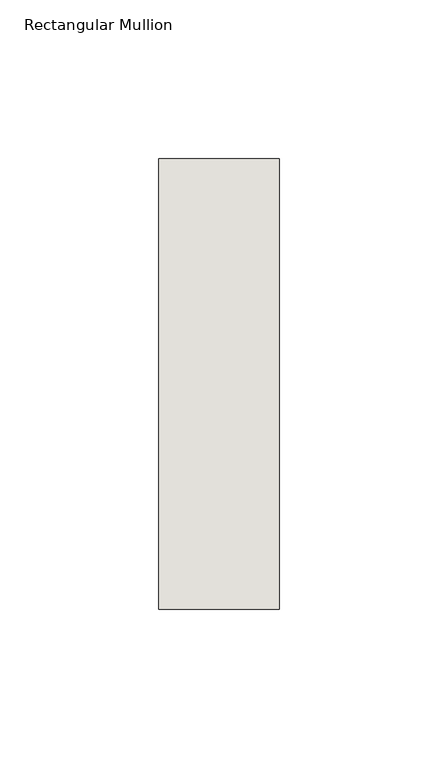
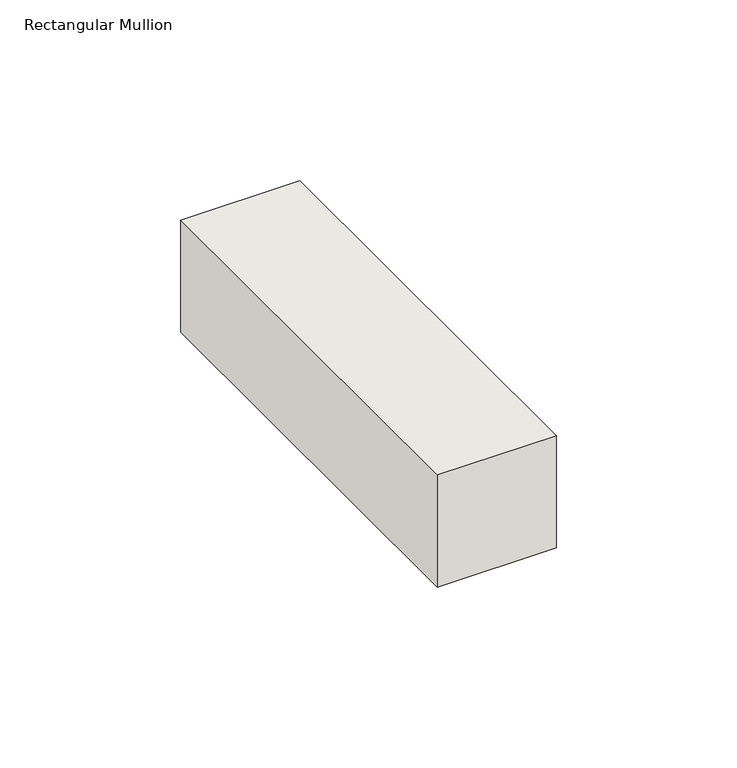
"""IFC4 building model written with IfcOpenShell, lengths in millimetres: wall geometry, Rectangular Mullion : NLRS_21_CWM_hsb-regel 38x142_gen_rsf."""

from ifc_helpers import new_model, si_unit, frame, origin, place, context, project, spatial, polyline, outline, extrude, source, transform, mapped, element, save


def rectangular_mullion_a2f1b024(model_context):
    return source(origin(), model_context, "Body", "SweptSolid", [
        extrude(outline(polyline([(0.0, -71.0), (-38.0, -71.0), (-38.0, 71.0), (0.0, 71.0), (0.0, -71.0)])), frame((0.0, 0.0, -38.0), z_axis=(0.0, 0.0, 1.0), x_axis=(1.0, 0.0, 0.0)), (0.0, 0.0, 1.0), 38.0),
    ])


if __name__ == "__main__":
    model = new_model("IFC4")
    model_context = context("Model", 3, world=origin())
    ifc_project = project(units=[si_unit("LENGTHUNIT", "METRE", prefix="MILLI")], contexts=[model_context])
    site = spatial("IfcSite", under=ifc_project)
    building = spatial("IfcBuilding", under=site)
    placement = place(None, origin())
    rectangular_mullion_shape = rectangular_mullion_a2f1b024(model_context)
    element("IfcWall", 1, ObjectType="Rectangular Mullion : NLRS_21_CWM_hsb-regel 38x142_gen_rsf", at=placement, inside=building, context=model_context, shape_type="MappedRepresentation", body=[
        mapped(rectangular_mullion_shape, transform((0.0, 0.0, 0.0), x_axis=(1.0, 0.0, 0.0), y_axis=(0.0, 1.0, 0.0), z_axis=(0.0, 0.0, 1.0))),
    ])
    save(model, "model.ifc")

# Revit data of these elements
# Type "Rectangular Mullion : NLRS_21_CWM_hsb-regel 38x142_gen_rsf"
#   Type IfcGUID = "07M7mRoiH1CR8m_RSKIwpF"
#   Assembly Code = "21.10"
#   IfcExportAs = "IfcWall"
#   built-in parameter 1007322 = 0.465879 (stored number, unit not read)
#   built-in parameter 1007321 = 0.062336 (stored number, unit not read)
#   built-in parameter 1007320 = 0.062336 (stored number, unit not read)
# Element 1 (IfcWall, "Rectangular Mullion : NLRS_21_CWM_hsb-regel 38x142_gen_rsf")
#   Materials on its faces: "NLRS_i2_hout naaldhout vuren_gen_rsf"
# Materials
#   "NLRS_i2_hout naaldhout vuren_gen_rsf": class "I - Hout", colour RGB 234 199 147, transparency 0, Keynote = "i2", Manufacturer = "Revit Standards Foundation", URL = "www.revitstandards.org", Description = "hout vuren", Cost = 0
